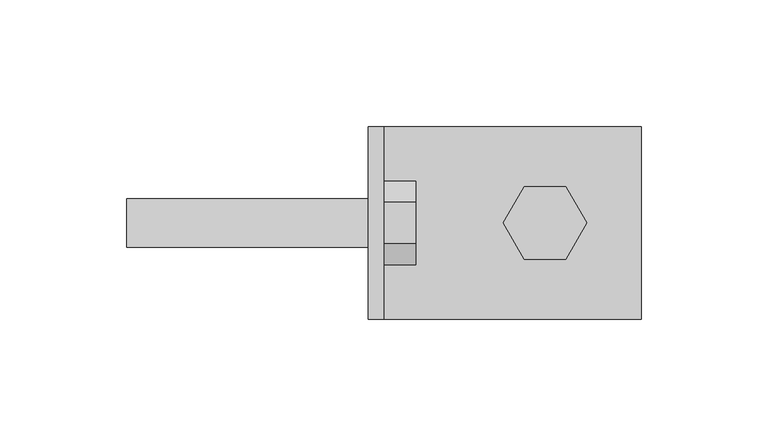
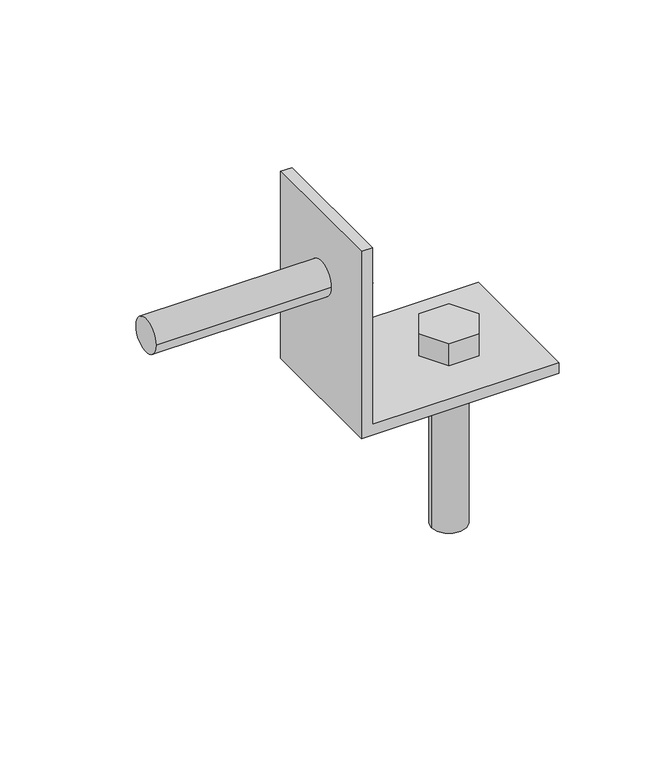
"""IFC4 building model written with IfcOpenShell, lengths in millimetres: fastener geometry, SIMPSON - HLPC/HLGPC Heavy Angles and Gussets : SIMPSON - HL43 - 3 X 4.25 - .75 Bolt - HDG."""

from ifc_helpers import new_model, si_unit, point, frame, frame_2d, origin, place, context, project, spatial, polyline, circle_curve, trimmed, segment, composite_curve, outline, extrude, source, transform, mapped, element, save
from ifc_brep_helpers import plane_surface, revolved_surface, advanced_brep


def fastener_b7801b40(model_context):
    return source(origin(), model_context, "Body", "SolidModel", [
        extrude(outline(composite_curve([segment(trimmed(circle_curve(frame_2d((0.0, 69.85)), 9.525), [point((9.525, 69.85))], [point((-9.525, 69.85))], False, "CARTESIAN"), True, "CONTINUOUS"), segment(trimmed(circle_curve(frame_2d((0.0, 69.85)), 9.525), [point((-9.525, 69.85))], [point((9.525, 69.85))], False, "CARTESIAN"), True, "CONTINUOUS")], self_intersect=False)), frame((-95.5476562, 0.0, 0.0), z_axis=(1.0, 0.0, 0.0), x_axis=(0.0, 1.0, 0.0)), (0.0, 0.0, 1.0), 101.6),
        extrude(outline(polyline([(16.4977839, 69.85), (8.248892, 55.5625), (-8.248892, 55.5625), (-16.4977839, 69.85), (-8.248892, 84.1375), (8.248892, 84.1375), (16.4977839, 69.85)])), frame((6.0523438, 0.0, 0.0), z_axis=(1.0, 0.0, 0.0), x_axis=(0.0, 1.0, 0.0)), (0.0, 0.0, 1.0), 12.7),
        extrude(outline(composite_curve([segment(trimmed(circle_curve(frame_2d((69.85, 0.0)), 9.525), [point((60.325, 0.0))], [point((79.375, 0.0))], False, "CARTESIAN"), True, "CONTINUOUS"), segment(trimmed(circle_curve(frame_2d((69.85, 0.0)), 9.525), [point((79.375, 0.0))], [point((60.325, 0.0))], False, "CARTESIAN"), True, "CONTINUOUS")], self_intersect=False)), frame((0.0, 0.0, -95.5476563), z_axis=(0.0, 0.0, 1.0), x_axis=(1.0, 0.0, 0.0)), (0.0, 0.0, 1.0), 101.6),
        extrude(outline(polyline([(53.3522161, 0.0), (61.601108, 14.2875), (78.098892, 14.2875), (86.3477839, 0.0), (78.098892, -14.2875), (61.601108, -14.2875), (53.3522161, 0.0)])), frame((0.0, 0.0, 6.0523437), z_axis=(0.0, 0.0, 1.0), x_axis=(1.0, 0.0, 0.0)), (0.0, 0.0, 1.0), 12.7),
        advanced_brep(
        [(6.0523438, -38.1, 107.95), (6.0523438, -38.1, 6.0523437), (6.0523438, 38.1, 6.0523437), (6.0523438, 38.1, 107.95), (6.0523438, -9.525, 69.85), (6.0523438, 9.525, 69.85), (0.0, 38.1, 107.95), (0.0, 38.1, 0.0), (0.0, -38.1, 0.0), (0.0, -38.1, 107.95), (0.0, 9.525, 69.85), (0.0, -9.525, 69.85), (107.95, 38.1, 6.0523437), (107.95, 38.1, 0.0), (107.95, -38.1, 0.0), (107.95, -38.1, 6.0523437), (79.375, 0.0, 6.0523437), (60.325, 0.0, 6.0523437), (60.325, 0.0, 0.0), (79.375, 0.0, 0.0)],
        [
            (0, 1),
            (1, 2),
            (2, 3),
            (3, 0),
            (4, 5, circle_curve(frame((6.0523438, 0.0, 69.85), z_axis=(-1.0, 0.0, 0.0), x_axis=(0.0, -1.0, 0.0)), 9.525)),
            (5, 4, circle_curve(frame((6.0523438, 0.0, 69.85), z_axis=(-1.0, 0.0, 0.0), x_axis=(0.0, -1.0, 0.0)), 9.525)),
            (6, 7),
            (7, 8),
            (8, 9),
            (9, 6),
            (10, 11, circle_curve(frame((0.0, 0.0, 69.85), z_axis=(1.0, 0.0, 0.0), x_axis=(0.0, -1.0, 0.0)), 9.525)),
            (11, 10, circle_curve(frame((0.0, 0.0, 69.85), z_axis=(1.0, 0.0, 0.0), x_axis=(0.0, -1.0, 0.0)), 9.525)),
            (3, 6),
            (9, 0),
            (2, 12),
            (12, 13),
            (13, 7),
            (8, 14),
            (14, 15),
            (15, 1),
            (15, 12),
            (16, 17, circle_curve(frame((69.85, 0.0, 6.0523437), z_axis=(0.0, 0.0, -1.0), x_axis=(1.0, 0.0, 0.0)), 9.525)),
            (17, 16, circle_curve(frame((69.85, 0.0, 6.0523437), z_axis=(0.0, 0.0, -1.0), x_axis=(1.0, 0.0, 0.0)), 9.525)),
            (13, 14),
            (18, 19, circle_curve(frame((69.85, 0.0, 0.0), z_axis=(0.0, 0.0, 1.0), x_axis=(1.0, 0.0, 0.0)), 9.525)),
            (19, 18, circle_curve(frame((69.85, 0.0, 0.0), z_axis=(0.0, 0.0, 1.0), x_axis=(1.0, 0.0, 0.0)), 9.525)),
            (17, 18),
            (19, 16),
            (5, 10),
            (11, 4),
        ],
        [
            plane_surface(frame((6.0523438, 38.1, 107.95), z_axis=(1.0, 0.0, 0.0), x_axis=(0.0, 1.0, 0.0))),
            plane_surface(frame((0.0, 38.1, 107.95), z_axis=(-1.0, 0.0, 0.0), x_axis=(0.0, -1.0, 0.0))),
            plane_surface(frame((6.0523438, -38.1, 107.95), z_axis=(0.0, 0.0, 1.0), x_axis=(-1.0, 0.0, 0.0))),
            plane_surface(frame((6.0523438, 38.1, 107.95), z_axis=(0.0, 1.0, 0.0), x_axis=(-1.0, 0.0, 0.0))),
            plane_surface(frame((6.0523438, -38.1, 6.0523437), z_axis=(0.0, -1.0, 0.0), x_axis=(-1.0, 0.0, 0.0))),
            plane_surface(frame((0.0, -38.1, 6.0523437), z_axis=(0.0, 0.0, 1.0), x_axis=(-1.0, 0.0, 0.0))),
            plane_surface(frame((0.0, -38.1, 0.0), z_axis=(0.0, 0.0, -1.0), x_axis=(1.0, 0.0, 0.0))),
            plane_surface(frame((107.95, 38.1, 6.0523437), z_axis=(1.0, 0.0, 0.0), x_axis=(0.0, 0.0, -1.0))),
            revolved_surface(polyline([(79.375, 0.0, 6.0523437), (79.375, 0.0, 0.0)]), (69.85, 0.0, 0.0), (0.0, 0.0, 1.0)),
            revolved_surface(polyline([(6.0523438, -9.525, 69.85), (0.0, -9.525, 69.85)]), (0.0, 0.0, 69.85), (1.0, 0.0, 0.0)),
        ],
        [
            (0, [[1, 2, 3, 4], [5, 6]]),
            (1, [[7, 8, 9, 10], [11, 12]]),
            (2, [[13, -10, 14, -4]]),
            (3, [[15, 16, 17, -7, -13, -3]]),
            (4, [[-14, -9, 18, 19, 20, -1]]),
            (5, [[-15, -2, -20, 21], [22, 23]]),
            (6, [[-18, -8, -17, 24], [25, 26]]),
            (7, [[-19, -24, -16, -21]]),
            (8, [[-23, 27, -26, 28]]),
            (8, [[-25, -27, -22, -28]]),
            (9, [[-6, 29, -12, 30]]),
            (9, [[-11, -29, -5, -30]]),
        ],
    ),
    ])


if __name__ == "__main__":
    model = new_model("IFC4")
    model_context = context("Model", 3, world=origin())
    ifc_project = project(units=[si_unit("LENGTHUNIT", "METRE", prefix="MILLI")], contexts=[model_context])
    site = spatial("IfcSite", under=ifc_project)
    building = spatial("IfcBuilding", under=site)
    placement = place(None, origin())
    fastener_shape = fastener_b7801b40(model_context)
    element("IfcFastener", 1, ObjectType="SIMPSON - HLPC/HLGPC Heavy Angles and Gussets : SIMPSON - HL43 - 3 X 4.25 - .75 Bolt - HDG", at=placement, inside=building, context=model_context, shape_type="MappedRepresentation", body=[
        mapped(fastener_shape, transform((0.0, 0.0, 0.0), x_axis=(1.0, 0.0, 0.0), y_axis=(0.0, 1.0, 0.0), z_axis=(0.0, 0.0, 1.0))),
    ])
    save(model, "model.ifc")

# Revit data of these elements
# Type "SIMPSON - HLPC/HLGPC Heavy Angles and Gussets : SIMPSON - HL43 - 3 X 4.25 - .75 Bolt - HDG"
#   URL = "https://www.strongtie.com/classiccollection_architecturalproductsgroup/hlpc-hlgpc_productgroup_wcc/p/hlpc.hlgpc"
#   L = 0' - 3"
#   Hole Radius = 0' - 0 3/8"
#   D4 = 0' - 5"
#   D2 = 0' - 5"
#   D1 = 0' - 1 1/2"
#   D3 = 0' - 2 3/4"
#   Ga. = 0' - 0 61/256"
#   W1 & W2 = 0' - 4 1/4"
#   Default Elevation = 4' - 0"
#   Bolt Visibility - 3B = no
#   Bolt Visibility - 3A = no
#   Bolt Visibility - 2B = no
#   Bolt Visibility - 2A = no
#   Bolt Visibility - 1B = no
#   Bolt Visibility - 1A = yes
#   Bolt Visibility = yes
#   Bolt Size = element 1298415
# Element 1 (IfcFastener, "SIMPSON - HLPC/HLGPC Heavy Angles and Gussets : SIMPSON - HL43 - 3 X 4.25 - .75 Bolt - HDG")
#   Materials on its faces: "1\" GALV. LAG BOLT (LENGTH = 1/2\" SHY OF GLULAM DEPTH) -  (GALV. THRU BOLT IF PLATE ON OPP. SIDE OF STRUCT MEMBER)"
# Materials
#   "1\" GALV. LAG BOLT (LENGTH = 1/2\" SHY OF GLULAM DEPTH) -  (GALV. THRU BOLT IF PLATE ON OPP. SIDE OF STRUCT MEMBER)": class "Generic", colour RGB 120 120 120, transparency 0, Cost = 0
